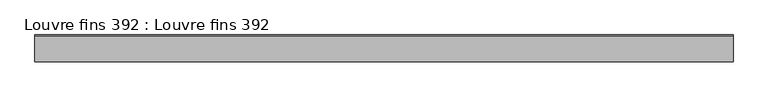
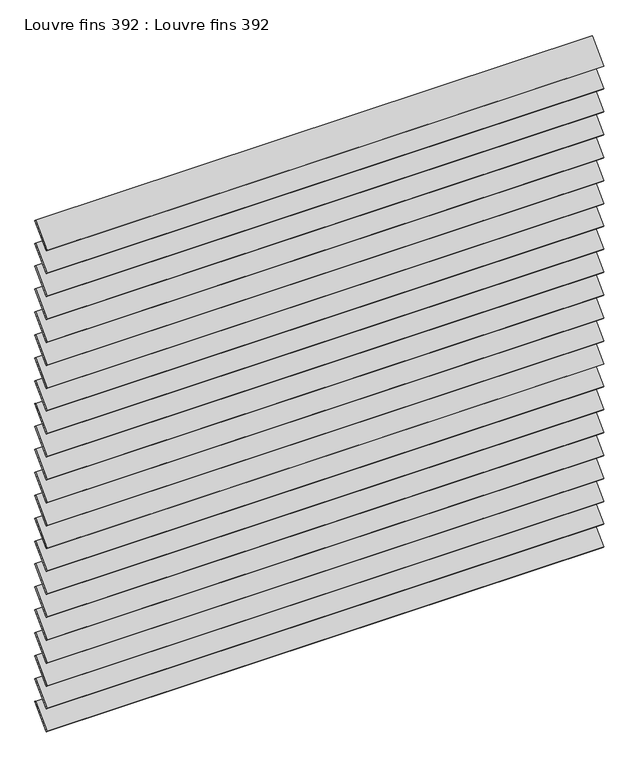
"""IFC4 building model written with IfcOpenShell, lengths in millimetres: proxy geometry, Louvre fins 392 : Louvre fins 392."""

import ifcopenshell
import ifcopenshell.guid

model = None  # the IFC model being written
_history = None  # IfcOwnerHistory: only IFC2X3 demands one
_inside = {}  # id of a spatial element -> (the spatial element, [elements in it])
_under = {}  # id of a project, library or spatial element -> (it, [spatial elements below it])
_declared = {}  # id of a project -> (the project, [libraries it declares])
_typed = {}  # id of a type object -> (the type object, [elements of that type])
_made_of = {}  # id of a material, layer set ... -> (it, [elements and type objects made of it])


def new_model(schema):
    """Start an empty IFC model of exactly this schema.

    Asked for "IFC4X3", IfcOpenShell would pick the latest addendum, in which some entities
    have other attributes; the version numbers below select the first issue.
    IFC2X3 requires an IfcOwnerHistory on every rooted entity: one is made here for all.
    """
    global model, _history
    if schema == "IFC4X3":
        model = ifcopenshell.file(schema_version=(4, 3, 0, 0))
    else:
        model = ifcopenshell.file(schema=schema)
    _inside.clear()
    _under.clear()
    _declared.clear()
    _typed.clear()
    _made_of.clear()
    _history = None
    if model.schema == "IFC2X3":
        org = make("IfcOrganization", Name="unknown")
        user = make(
            "IfcPersonAndOrganization",
            ThePerson=make("IfcPerson", FamilyName="unknown"),
            TheOrganization=org,
        )
        app = make(
            "IfcApplication",
            ApplicationDeveloper=org,
            Version="unknown",
            ApplicationFullName="unknown",
            ApplicationIdentifier="unknown",
        )
        _history = make(
            "IfcOwnerHistory",
            OwningUser=user,
            OwningApplication=app,
            ChangeAction="ADDED",
            CreationDate=0,
        )
    return model


def make(cls, **values):
    """One entity of the class cls with the attributes given. An attribute that is None is left unset."""
    return model.create_entity(
        cls, **{name: value for name, value in values.items() if value is not None}
    )


def rooted(cls, **values):
    """An entity with a GlobalId (a new one), such as an element, a storey or a relation."""
    return make(cls, GlobalId=ifcopenshell.guid.new(), OwnerHistory=_history, **values)


def si_unit(unit_type, name, prefix=None):
    """IfcSIUnit, for example si_unit("LENGTHUNIT", "METRE", prefix="MILLI")."""
    return make("IfcSIUnit", UnitType=unit_type, Prefix=prefix, Name=name)


def assignment(units):
    """IfcUnitAssignment: the units of a project."""
    return None if units is None else make("IfcUnitAssignment", Units=units)


def point(xyz):
    """IfcCartesianPoint."""
    return None if xyz is None else make("IfcCartesianPoint", Coordinates=xyz)


def direction(xyz):
    """IfcDirection."""
    return None if xyz is None else make("IfcDirection", DirectionRatios=xyz)


def frame(location, z_axis=None, x_axis=None):
    """IfcAxis2Placement3D, a coordinate frame: its origin and axes. An axis left out is left unset."""
    return make(
        "IfcAxis2Placement3D",
        Location=point(location),
        Axis=direction(z_axis),
        RefDirection=direction(x_axis),
    )


def origin():
    """The frame at (0, 0, 0) with its axes left unset."""
    return frame((0.0, 0.0, 0.0))


def place(relative_to, where):
    """IfcLocalPlacement: puts the frame where relative to a parent placement (None: the world)."""
    return make(
        "IfcLocalPlacement", PlacementRelTo=relative_to, RelativePlacement=where
    )


def context(
    kind, dimensions, precision=None, world=None, true_north=None, identifier=None
):
    """IfcGeometricRepresentationContext, for example the 3D "Model" context."""
    return make(
        "IfcGeometricRepresentationContext",
        ContextIdentifier=identifier,
        ContextType=kind,
        CoordinateSpaceDimension=dimensions,
        Precision=precision,
        WorldCoordinateSystem=world,
        TrueNorth=true_north,
    )


def project(units=None, contexts=None):
    """IfcProject with its units and contexts."""
    return rooted(
        "IfcProject",
        Name="project",
        RepresentationContexts=contexts,
        UnitsInContext=assignment(units),
    )


def spatial(cls, under=None, at=None, **own):
    """A site, building, storey or space (cls), placed at a placement, below another one or the project."""
    s = rooted(cls, ObjectPlacement=at, **own)
    if under is not None:
        _under.setdefault(under.id(), (under, []))[1].append(s)
    return s


def polyline(points):
    """IfcPolyline through the points."""
    return make("IfcPolyline", Points=[point(p) for p in points])


def outline(outer, holes=None, kind="AREA"):
    """IfcArbitraryClosedProfileDef: a profile drawn as a closed curve; with holes, ...WithVoids."""
    if holes is None:
        return make("IfcArbitraryClosedProfileDef", ProfileType=kind, OuterCurve=outer)
    return make(
        "IfcArbitraryProfileDefWithVoids",
        ProfileType=kind,
        OuterCurve=outer,
        InnerCurves=holes,
    )


def extrude(swept, where, along, depth):
    """IfcExtrudedAreaSolid: the profile swept, set in the frame where, extruded along a direction by depth."""
    return make(
        "IfcExtrudedAreaSolid",
        SweptArea=swept,
        Position=where,
        ExtrudedDirection=direction(along),
        Depth=depth,
    )


def shape(context_of_items, identifier, shape_type, items):
    """IfcShapeRepresentation: the items that make up one representation, for example the "Body"."""
    return make(
        "IfcShapeRepresentation",
        ContextOfItems=context_of_items,
        RepresentationIdentifier=identifier,
        RepresentationType=shape_type,
        Items=items,
    )


def source(mapping_origin, context_of_items, identifier, shape_type, items):
    """IfcRepresentationMap: a shape defined once, which mapped items show again and again."""
    return make(
        "IfcRepresentationMap",
        MappingOrigin=mapping_origin,
        MappedRepresentation=shape(context_of_items, identifier, shape_type, items),
    )


def transform(
    local_origin,
    x_axis=None,
    y_axis=None,
    z_axis=None,
    scale=None,
    scale2=None,
    scale3=None,
    uniform=True,
):
    """IfcCartesianTransformationOperator3D, or its non-uniform kind. x_axis, y_axis, z_axis: its Axis1, 2, 3."""
    if uniform:
        return make(
            "IfcCartesianTransformationOperator3D",
            Axis1=direction(x_axis),
            Axis2=direction(y_axis),
            LocalOrigin=point(local_origin),
            Scale=scale,
            Axis3=direction(z_axis),
        )
    return make(
        "IfcCartesianTransformationOperator3DnonUniform",
        Axis1=direction(x_axis),
        Axis2=direction(y_axis),
        LocalOrigin=point(local_origin),
        Scale=scale,
        Axis3=direction(z_axis),
        Scale2=scale2,
        Scale3=scale3,
    )


def mapped(mapping_source, mapping_target):
    """IfcMappedItem: shows the shape of a source again, moved by a transform."""
    return make(
        "IfcMappedItem", MappingSource=mapping_source, MappingTarget=mapping_target
    )


def made_of(thing, what):
    """Note that an element or type object is made of a material, layer set ...; save() writes the relation."""
    if what is not None:
        _made_of.setdefault(what.id(), (what, []))[1].append(thing)
    return thing


def element(
    cls,
    number,
    at=None,
    inside=None,
    cuts=None,
    type_object=None,
    material=None,
    context=None,
    identifier="Body",
    shape_type=None,
    held_by="IfcProductDefinitionShape",
    body=None,
    shapes=None,
    **own,
):
    """One element of the class cls, such as IfcWall. Its Tag is "e" and its number.

    at: its placement. inside: the storey or other place that contains it. cuts: it is an
    opening in that element (IfcRelVoidsElement). A single representation is given by context,
    identifier, shape_type and body (its items); several are given by shapes. held_by: the class
    of the entity that holds the representations. save() writes the other relations.
    """
    e = rooted(cls, Tag="e%d" % number, ObjectPlacement=at, **own)
    if body is not None:
        shapes = [shape(context, identifier, shape_type, body)]
    if shapes is not None:
        e.Representation = make(held_by, Representations=shapes)
    if inside is not None:
        _inside.setdefault(inside.id(), (inside, []))[1].append(e)
    if cuts is not None:
        rooted(
            "IfcRelVoidsElement", RelatingBuildingElement=cuts, RelatedOpeningElement=e
        )
    if type_object is not None:
        _typed.setdefault(type_object.id(), (type_object, []))[1].append(e)
    return made_of(e, material)


def aggregate(whole, parts):
    """IfcRelAggregates: a whole, such as a stair, and the parts it consists of."""
    return rooted("IfcRelAggregates", RelatingObject=whole, RelatedObjects=parts)


def save(model, path):
    """Write the relations noted so far, then the file.

    IfcRelAggregates (storeys below a building ...), IfcRelContainedInSpatialStructure (elements
    in a storey), IfcRelDefinesByType, IfcRelAssociatesMaterial and IfcRelDeclares: one each for
    every whole, place, type object, material and project.
    """
    for whole, parts in _under.values():
        aggregate(whole, parts)
    for where, things in _inside.values():
        rooted(
            "IfcRelContainedInSpatialStructure",
            RelatedElements=things,
            RelatingStructure=where,
        )
    for kind, things in _typed.values():
        rooted("IfcRelDefinesByType", RelatedObjects=things, RelatingType=kind)
    for what, things in _made_of.values():
        rooted("IfcRelAssociatesMaterial", RelatedObjects=things, RelatingMaterial=what)
    for by, libraries in _declared.values():
        rooted("IfcRelDeclares", RelatingContext=by, RelatedDefinitions=libraries)
    model.write(path)


def louvre_fins_392_louvre_fins_392_fe2ccf94(model_context):
    return source(origin(), model_context, "Body", "SweptSolid", [
        extrude(outline(polyline([(0.0, -6.35), (0.0, 0.0), (2000.0, 0.0), (2000.0, -6.35), (0.0, -6.35)])), frame((3694.2883192, 9806.3460022, 37559.769849), z_axis=(0.0, 0.707106781186377, 0.7071067811867181), x_axis=(1.0, 0.0, 0.0)), (0.0, 0.0, 1.0), 101.6),
        extrude(outline(polyline([(0.0, -6.35), (0.0, 0.0), (2000.0, 0.0), (2000.0, -6.35), (0.0, -6.35)])), frame((3694.2883192, 9806.3460022, 37646.769849), z_axis=(0.0, 0.707106781186377, 0.7071067811867181), x_axis=(1.0, 0.0, 0.0)), (0.0, 0.0, 1.0), 101.6),
        extrude(outline(polyline([(0.0, -6.35), (0.0, 0.0), (2000.0, 0.0), (2000.0, -6.35), (0.0, -6.35)])), frame((3694.2883192, 9806.3460022, 37733.769849), z_axis=(0.0, 0.707106781186377, 0.7071067811867181), x_axis=(1.0, 0.0, 0.0)), (0.0, 0.0, 1.0), 101.6),
        extrude(outline(polyline([(0.0, -6.35), (0.0, 0.0), (2000.0, 0.0), (2000.0, -6.35), (0.0, -6.35)])), frame((3694.2883192, 9806.3460022, 37820.769849), z_axis=(0.0, 0.707106781186377, 0.7071067811867181), x_axis=(1.0, 0.0, 0.0)), (0.0, 0.0, 1.0), 101.6),
        extrude(outline(polyline([(0.0, -6.35), (0.0, 0.0), (2000.0, 0.0), (2000.0, -6.35), (0.0, -6.35)])), frame((3694.2883192, 9806.3460022, 37907.769849), z_axis=(0.0, 0.7071067811865476, 0.7071067811865476), x_axis=(1.0, 0.0, 0.0)), (0.0, 0.0, 1.0), 101.6),
        extrude(outline(polyline([(0.0, -6.35), (0.0, 0.0), (2000.0, 0.0), (2000.0, -6.35), (0.0, -6.35)])), frame((3694.2883192, 9806.3460022, 37994.769849), z_axis=(0.0, 0.707106781186377, 0.7071067811867181), x_axis=(1.0, 0.0, 0.0)), (0.0, 0.0, 1.0), 101.6),
        extrude(outline(polyline([(0.0, -6.35), (0.0, 0.0), (2000.0, 0.0), (2000.0, -6.35), (0.0, -6.35)])), frame((3694.2883192, 9806.3460022, 38081.769849), z_axis=(0.0, 0.7071067811865476, 0.7071067811865476), x_axis=(1.0, 0.0, 0.0)), (0.0, 0.0, 1.0), 101.6),
        extrude(outline(polyline([(0.0, -6.35), (0.0, 0.0), (2000.0, 0.0), (2000.0, -6.35), (0.0, -6.35)])), frame((3694.2883192, 9806.3460022, 38168.769849), z_axis=(0.0, 0.707106781186377, 0.7071067811867181), x_axis=(1.0, 0.0, 0.0)), (0.0, 0.0, 1.0), 101.6),
        extrude(outline(polyline([(0.0, -6.35), (0.0, 0.0), (2000.0, 0.0), (2000.0, -6.35), (0.0, -6.35)])), frame((3694.2883192, 9806.3460022, 38255.769849), z_axis=(0.0, 0.7071067811865476, 0.7071067811865476), x_axis=(1.0, 0.0, 0.0)), (0.0, 0.0, 1.0), 101.6),
        extrude(outline(polyline([(0.0, -6.35), (0.0, 0.0), (2000.0, 0.0), (2000.0, -6.35), (0.0, -6.35)])), frame((3694.2883192, 9806.3460022, 38342.769849), z_axis=(0.0, 0.707106781186377, 0.7071067811867181), x_axis=(1.0, 0.0, 0.0)), (0.0, 0.0, 1.0), 101.6),
        extrude(outline(polyline([(0.0, -6.35), (0.0, 0.0), (2000.0, 0.0), (2000.0, -6.35), (0.0, -6.35)])), frame((3694.2883192, 9806.3460022, 38429.769849), z_axis=(0.0, 0.7071067811868886, 0.7071067811862065), x_axis=(1.0, 0.0, 0.0)), (0.0, 0.0, 1.0), 101.6),
        extrude(outline(polyline([(0.0, -6.35), (0.0, 0.0), (2000.0, 0.0), (2000.0, -6.35), (0.0, -6.35)])), frame((3694.2883192, 9806.3460022, 38516.769849), z_axis=(0.0, 0.707106781186377, 0.7071067811867181), x_axis=(1.0, 0.0, 0.0)), (0.0, 0.0, 1.0), 101.6),
        extrude(outline(polyline([(0.0, -6.35), (0.0, 0.0), (2000.0, 0.0), (2000.0, -6.35), (0.0, -6.35)])), frame((3694.2883192, 9806.3460022, 38603.769849), z_axis=(0.0, 0.707106781186377, 0.7071067811867181), x_axis=(1.0, 0.0, 0.0)), (0.0, 0.0, 1.0), 101.6),
        extrude(outline(polyline([(0.0, -6.35), (0.0, 0.0), (2000.0, 0.0), (2000.0, -6.35), (0.0, -6.35)])), frame((3694.2883192, 9806.3460022, 38690.769849), z_axis=(0.0, 0.707106781186377, 0.7071067811867181), x_axis=(1.0, 0.0, 0.0)), (0.0, 0.0, 1.0), 101.6),
        extrude(outline(polyline([(0.0, -6.35), (0.0, 0.0), (2000.0, 0.0), (2000.0, -6.35), (0.0, -6.35)])), frame((3694.2883192, 9806.3460022, 38777.769849), z_axis=(0.0, 0.7071067811868886, 0.7071067811862065), x_axis=(1.0, 0.0, 0.0)), (0.0, 0.0, 1.0), 101.6),
        extrude(outline(polyline([(0.0, -6.35), (0.0, 0.0), (2000.0, 0.0), (2000.0, -6.35), (0.0, -6.35)])), frame((3694.2883192, 9806.3460022, 38864.769849), z_axis=(0.0, 0.707106781186377, 0.7071067811867181), x_axis=(1.0, 0.0, 0.0)), (0.0, 0.0, 1.0), 101.6),
        extrude(outline(polyline([(0.0, -6.35), (0.0, 0.0), (2000.0, 0.0), (2000.0, -6.35), (0.0, -6.35)])), frame((3694.2883192, 9806.3460022, 38951.769849), z_axis=(0.0, 0.7071067811867181, 0.707106781186377), x_axis=(1.0, 0.0, 0.0)), (0.0, 0.0, 1.0), 101.6),
        extrude(outline(polyline([(0.0, -6.35), (0.0, 0.0), (2000.0, 0.0), (2000.0, -6.35), (0.0, -6.35)])), frame((3694.2883192, 9806.3460022, 39038.769849), z_axis=(0.0, 0.707106781186036, 0.7071067811870592), x_axis=(1.0, 0.0, 0.0)), (0.0, 0.0, 1.0), 101.6),
        extrude(outline(polyline([(0.0, -6.35), (0.0, 0.0), (2000.0, 0.0), (2000.0, -6.35), (0.0, -6.35)])), frame((3694.2883192, 9806.3460022, 39125.769849), z_axis=(0.0, 0.7071067811862065, 0.7071067811868886), x_axis=(1.0, 0.0, 0.0)), (0.0, 0.0, 1.0), 101.6),
        extrude(outline(polyline([(0.0, -6.35), (0.0, 0.0), (2000.0, 0.0), (2000.0, -6.35), (0.0, -6.35)])), frame((3694.2883192, 9806.3460022, 39212.769849), z_axis=(0.0, 0.7071067811868886, 0.7071067811862065), x_axis=(1.0, 0.0, 0.0)), (0.0, 0.0, 1.0), 101.6),
        extrude(outline(polyline([(0.0, -6.35), (0.0, 0.0), (2000.0, 0.0), (2000.0, -6.35), (0.0, -6.35)])), frame((3694.2883192, 9806.3460022, 39299.769849), z_axis=(0.0, 0.7071067811865476, 0.7071067811865476), x_axis=(1.0, 0.0, 0.0)), (0.0, 0.0, 1.0), 101.6),
        extrude(outline(polyline([(0.0, -6.35), (0.0, 0.0), (2000.0, 0.0), (2000.0, -6.35), (0.0, -6.35)])), frame((3694.2883192, 9806.3460022, 39386.769849), z_axis=(0.0, 0.7071067811862065, 0.7071067811868886), x_axis=(1.0, 0.0, 0.0)), (0.0, 0.0, 1.0), 101.6),
    ])


if __name__ == "__main__":
    model = new_model("IFC4")
    model_context = context("Model", 3, world=origin())
    ifc_project = project(units=[si_unit("LENGTHUNIT", "METRE", prefix="MILLI")], contexts=[model_context])
    site = spatial("IfcSite", under=ifc_project)
    building = spatial("IfcBuilding", under=site)
    placement = place(None, origin())
    louvre_fins_392_louvre_fins_392_shape = louvre_fins_392_louvre_fins_392_fe2ccf94(model_context)
    element("IfcBuildingElementProxy", 1, Name="Louvre fins 392 : Louvre fins 392", ObjectType="Louvre fins 392 : Louvre fins 392", at=placement, inside=building, context=model_context, shape_type="MappedRepresentation", body=[
        mapped(louvre_fins_392_louvre_fins_392_shape, transform((0.0, 0.0, 0.0), x_axis=(1.0, 0.0, 0.0), y_axis=(0.0, 1.0, 0.0), z_axis=(0.0, 0.0, 1.0))),
    ])
    save(model, "model.ifc")

# Revit data of these elements
# Type "Louvre fins 392 : Louvre fins 392"
#   NameOverride = "Louvre fins"
# Element 1 (IfcBuildingElementProxy, "Louvre fins 392 : Louvre fins 392")
#   Materials on its faces: "ALUMINIUM LOUVRE - TBD"
# Materials
#   "ALUMINIUM LOUVRE - TBD": class "Unassigned", colour RGB 92 107 122, transparency 0
